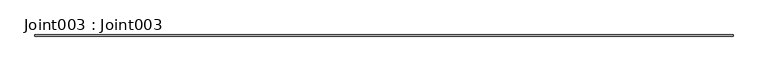
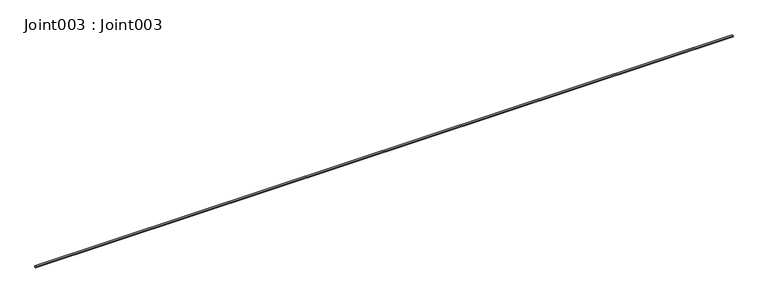
"""IFC4 building model written with IfcOpenShell, lengths in millimetres: proxy geometry, Joint003 : Joint003."""

from ifc_helpers import new_model, si_unit, point, frame, frame_2d, origin, place, context, project, spatial, polyline, circle_curve, trimmed, segment, composite_curve, outline, extrude, source, transform, mapped, element, save


def joint003_joint003_9bc8abc8(model_context):
    return source(origin(), model_context, "Body", "SweptSolid", [
        extrude(outline(composite_curve([segment(polyline([(9721.6885026, 39516.5389688), (9721.6885026, 39512.621)]), True, "CONTINUOUS"), segment(trimmed(circle_curve(frame_2d((9720.0901706, 39507.449125)), 5.4132205), [point((9721.6885026, 39512.621))], [point((9718.4918386, 39512.621))], True, "CARTESIAN"), True, "CONTINUOUS"), segment(polyline([(9718.4918386, 39512.621), (9718.4918386, 39516.5389688)]), True, "CONTINUOUS"), segment(trimmed(circle_curve(frame_2d((9720.0901706, 39511.3670938)), 5.4132205), [point((9718.4918386, 39516.5389688))], [point((9721.6885026, 39516.5389688))], False, "CARTESIAN"), True, "CONTINUOUS")], self_intersect=False)), frame((3694.2883192, 0.0, 0.0), z_axis=(1.0, 0.0, 0.0), x_axis=(0.0, 1.0, 0.0)), (0.0, 0.0, 1.0), 2000.0),
    ])


if __name__ == "__main__":
    model = new_model("IFC4")
    model_context = context("Model", 3, world=origin())
    ifc_project = project(units=[si_unit("LENGTHUNIT", "METRE", prefix="MILLI")], contexts=[model_context])
    site = spatial("IfcSite", under=ifc_project)
    building = spatial("IfcBuilding", under=site)
    placement = place(None, origin())
    joint003_joint003_shape = joint003_joint003_9bc8abc8(model_context)
    element("IfcBuildingElementProxy", 1, Name="Joint003 : Joint003", ObjectType="Joint003 : Joint003", at=placement, inside=building, context=model_context, shape_type="MappedRepresentation", body=[
        mapped(joint003_joint003_shape, transform((0.0, 0.0, 0.0), x_axis=(1.0, 0.0, 0.0), y_axis=(0.0, 1.0, 0.0), z_axis=(0.0, 0.0, 1.0))),
    ])
    save(model, "model.ifc")

# Revit data of these elements
# Type "Joint003 : Joint003"
#   NameOverride = "Joint003"
# Element 1 (IfcBuildingElementProxy, "Joint003 : Joint003")
#   Materials on its faces: "SEALANT JOINT"
# Materials
#   "SEALANT JOINT": class "Unassigned", colour RGB 142 225 148, transparency 0
